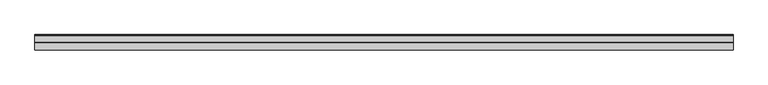
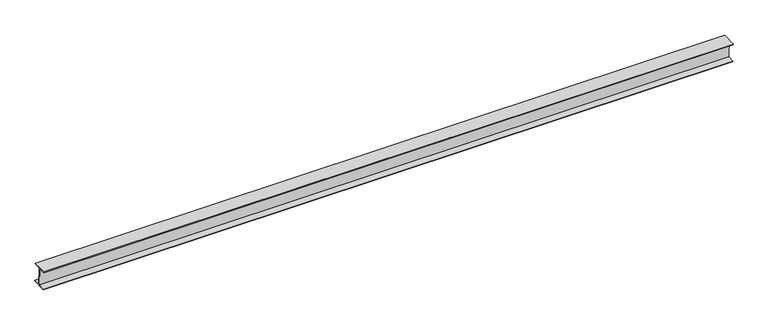
"""IFC4 building model written with IfcOpenShell, lengths in millimetres: proxy geometry, Generic Models 7:Generic Models 1:8:Generic Models 1:8 : Generic Models 7:Generic Models 1:337419:40 : Generic Models 7:Generic Models 1:8:Generic Models 1:8 : Generic Models 7:Generic Models 1:337419:315935."""

from ifc_helpers import new_model, si_unit, frame, origin, place, context, project, spatial, polyline, outline, extrude, source, transform, mapped, element, save


def generic_models_2f5065d5(model_context):
    return source(origin(), model_context, "Body", "SweptSolid", [
        extrude(outline(polyline([(-576429.5235686, 4024.8210459), (-576429.7959773, 4031.6736335), (-576277.5162517, 4037.7271598), (-576277.243843, 4030.8745722), (-576350.4650111, 4027.963835), (-576342.93846, 3838.6293762), (-576269.7357554, 3841.5393794), (-576269.4633467, 3834.6867918), (-576421.7430723, 3828.6332655), (-576422.015481, 3835.4858531), (-576349.0296491, 3838.3872351), (-576356.5562001, 4027.7216939), (-576429.5235686, 4024.8210459)])), frame((659949.5367238, 0.0, 0.0), z_axis=(1.0, 0.0, 0.0), x_axis=(0.0, 1.0, 0.0)), (0.0, 0.0, 1.0), 7315.2),
    ])


if __name__ == "__main__":
    model = new_model("IFC4")
    model_context = context("Model", 3, world=origin())
    ifc_project = project(units=[si_unit("LENGTHUNIT", "METRE", prefix="MILLI")], contexts=[model_context])
    site = spatial("IfcSite", under=ifc_project)
    building = spatial("IfcBuilding", under=site)
    placement = place(None, origin())
    generic_models_shape = generic_models_2f5065d5(model_context)
    element("IfcBuildingElementProxy", 1, Name="Generic Models 7:Generic Models 1:8:Generic Models 1:8 : Generic Models 7:Generic Models 1:337419:40 : Generic Models 7:Generic Models 1:8:Generic Models 1:8 : Generic Models 7:Generic Models 1:337419:315935", ObjectType="Generic Models 7:Generic Models 1:8:Generic Models 1:8 : Generic Models 7:Generic Models 1:337419:40 : Generic Models 7:Generic Models 1:8:Generic Models 1:8 : Generic Models 7:Generic Models 1:337419:315935", at=placement, inside=building, context=model_context, shape_type="MappedRepresentation", body=[
        mapped(generic_models_shape, transform((0.0, 0.0, 0.0), x_axis=(1.0, 0.0, 0.0), y_axis=(0.0, 1.0, 0.0), z_axis=(0.0, 0.0, 1.0))),
    ])
    save(model, "model.ifc")

# Revit data of these elements
# Type "Generic Models 7:Generic Models 1:8:Generic Models 1:8 : Generic Models 7:Generic Models 1:337419:40 : Generic Models 7:Generic Models 1:8:Generic Models 1:8 : Generic Models 7:Generic Models 1:337419:315935"
#   NameOverride = "Generic Models 7:Generic Models 1:8:Generic Models 1:8 : Generic Models 7:Generic Models 1:337419:315935"
#   ObjectTypeOverride = "Generic Models 1:8 : Generic Models 7:Generic Models 1:337419"
#   Reference = "Generic Models 1"
#   Tag = "315935"
# Element 1 (IfcBuildingElementProxy, "Generic Models 7:Generic Models 1:8:Generic Models 1:8 : Generic Models 7:Generic Models 1:337419:40 : Generic Models 7:Generic Models 1:8:Generic Models 1:8 : Generic Models 7:Generic Models 1:337419:315935")
#   Materials on its faces: "STRUCTURAL STEEL - SEE STRUCT. DWGS"
# Materials
#   "STRUCTURAL STEEL - SEE STRUCT. DWGS": class "Metal", colour RGB 189 187 185, transparency 0, Description = "Structural steel 50ksi", Cost = 0
